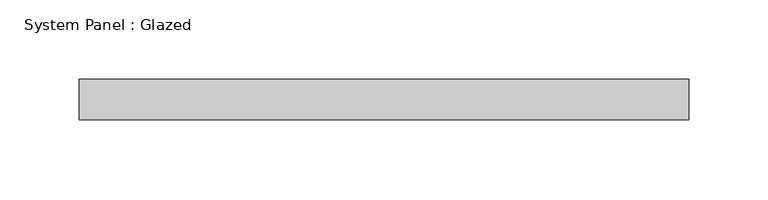
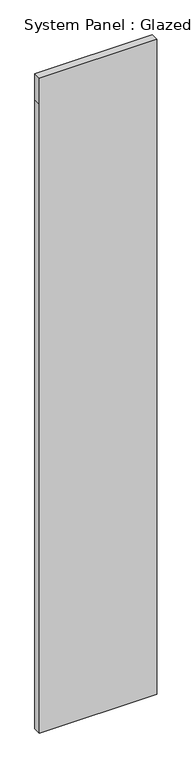
"""IFC4 building model written with IfcOpenShell, lengths in millimetres: plate geometry, System Panel : Glazed."""

from ifc_helpers import new_model, si_unit, frame, origin, place, context, project, spatial, polyline, outline, extrude, source, transform, mapped, element, save


def system_panel_glazed_cf7dde91(model_context):
    return source(origin(), model_context, "Body", "SweptSolid", [
        extrude(outline(polyline([(0.0, -191.6975988), (0.0, 191.6975988), (2171.7, 191.6975988), (2260.6, 191.6975988), (2260.6, -191.6975988), (2171.7, -191.6975988), (0.0, -191.6975988)])), frame((0.0, 19.05, 0.0), z_axis=(0.0, 1.0, 0.0), x_axis=(0.0, 0.0, 1.0)), (0.0, 0.0, 1.0), 25.4),
    ])


if __name__ == "__main__":
    model = new_model("IFC4")
    model_context = context("Model", 3, world=origin())
    ifc_project = project(units=[si_unit("LENGTHUNIT", "METRE", prefix="MILLI")], contexts=[model_context])
    site = spatial("IfcSite", under=ifc_project)
    building = spatial("IfcBuilding", under=site)
    placement = place(None, origin())
    system_panel_glazed_shape = system_panel_glazed_cf7dde91(model_context)
    element("IfcPlate", 1, ObjectType="System Panel : Glazed", at=placement, inside=building, context=model_context, shape_type="MappedRepresentation", body=[
        mapped(system_panel_glazed_shape, transform((0.0, 0.0, 0.0), x_axis=(1.0, 0.0, 0.0), y_axis=(0.0, 1.0, 0.0), z_axis=(0.0, 0.0, 1.0))),
    ])
    save(model, "model.ifc")

# Revit data of these elements
# Element 1 (IfcPlate, "System Panel : Glazed")
#   Materials on its faces: "Glass"
# Materials
#   "Glass": class "Glass", colour RGB 218 227 224, transparency 0.85, Description = "Soda Lime Glass", Cost = 0
